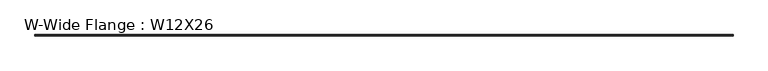
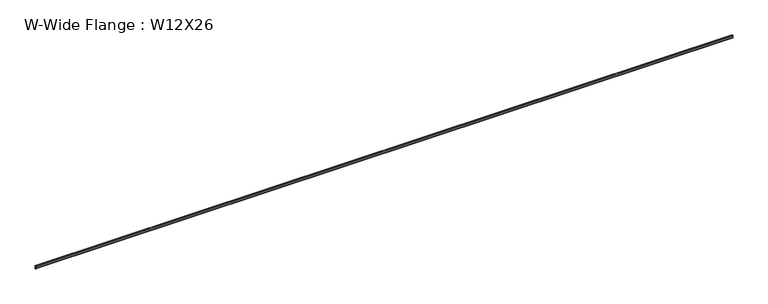
"""IFC4 building model written with IfcOpenShell, lengths in millimetres: beam geometry, W-Wide Flange : W12X26."""

from ifc_helpers import new_model, si_unit, point, frame, frame_2d, origin, place, context, project, spatial, polyline, circle_curve, trimmed, segment, composite_curve, outline, extrude, source, transform, mapped, element, save


def w_wide_flange_w12x26_e8f2a0f4(model_context):
    return source(origin(), model_context, "Body", "SweptSolid", [
        extrude(outline(composite_curve([segment(polyline([(82.4011719, -145.5539063), (82.4011719, -155.178125), (-82.4011719, -155.178125), (-82.4011719, -145.5539063), (-20.2902344, -145.5539063)]), True, "CONTINUOUS"), segment(trimmed(circle_curve(frame_2d((-20.2902344, -128.190625)), 17.3632812), [point((-20.2902344, -145.5539063))], [point((-2.9269531, -128.190625))], True, "CARTESIAN"), True, "CONTINUOUS"), segment(polyline([(-2.9269531, -128.190625), (-2.9269531, 128.190625)]), True, "CONTINUOUS"), segment(trimmed(circle_curve(frame_2d((-20.2902344, 128.190625)), 17.3632812), [point((-2.9269531, 128.190625))], [point((-20.2902344, 145.5539062))], True, "CARTESIAN"), True, "CONTINUOUS"), segment(polyline([(-20.2902344, 145.5539062), (-82.4011719, 145.5539062), (-82.4011719, 155.178125), (82.4011719, 155.178125), (82.4011719, 145.5539062), (20.2902344, 145.5539062)]), True, "CONTINUOUS"), segment(trimmed(circle_curve(frame_2d((20.2902344, 128.190625)), 17.3632812), [point((20.2902344, 145.5539062))], [point((2.9269531, 128.190625))], True, "CARTESIAN"), True, "CONTINUOUS"), segment(polyline([(2.9269531, 128.190625), (2.9269531, -128.190625)]), True, "CONTINUOUS"), segment(trimmed(circle_curve(frame_2d((20.2902344, -128.190625)), 17.3632812), [point((2.9269531, -128.190625))], [point((20.2902344, -145.5539063))], True, "CARTESIAN"), True, "CONTINUOUS"), segment(polyline([(20.2902344, -145.5539063), (82.4011719, -145.5539063)]), True, "CONTINUOUS")], self_intersect=False)), frame((-45384.7199999, 0.0, 0.0), z_axis=(1.0, 0.0, 0.0), x_axis=(0.0, 1.0, 0.0)), (0.0, 0.0, 1.0), 90769.4400002),
    ])


if __name__ == "__main__":
    model = new_model("IFC4")
    model_context = context("Model", 3, world=origin())
    ifc_project = project(units=[si_unit("LENGTHUNIT", "METRE", prefix="MILLI")], contexts=[model_context])
    site = spatial("IfcSite", under=ifc_project)
    building = spatial("IfcBuilding", under=site)
    placement = place(None, origin())
    w_wide_flange_w12x26_shape = w_wide_flange_w12x26_e8f2a0f4(model_context)
    element("IfcBeam", 1, ObjectType="W-Wide Flange : W12X26", at=placement, inside=building, context=model_context, shape_type="MappedRepresentation", body=[
        mapped(w_wide_flange_w12x26_shape, transform((0.0, 0.0, 0.0), x_axis=(1.0, 0.0, 0.0), y_axis=(0.0, 1.0, 0.0), z_axis=(0.0, 0.0, 1.0))),
    ])
    save(model, "model.ifc")

# Revit data of these elements
# Type "W-Wide Flange : W12X26"
#   Assembly Code = "B10"
#   W = 26
#   Length [instance default] = 5' - 0"
#   bf = 0' - 6 125/256"
#   d = 1' - 0 7/32"
#   k = 0' - 1 1/16"
#   k2 = 0' - 0 175/256"
#   tf = 0' - 0 97/256"
#   tw = 0' - 0 59/256"
#   A = 0.053125 SF
#   Structural Material [instance default] = Steel ASTM A992
# Element 1 (IfcBeam, "W-Wide Flange : W12X26")
#   Structural Material = Steel
#   Materials on its faces: "Steel"
# Materials
#   "Steel ASTM A992": class "Metal", colour RGB 199 199 199, transparency 0, Description = "Structural steel 50ksi", Cost = 0
#   "Steel": class "Metal", colour RGB 118 118 114, transparency 0, Description = "Steel, mill finish", Cost = 0
